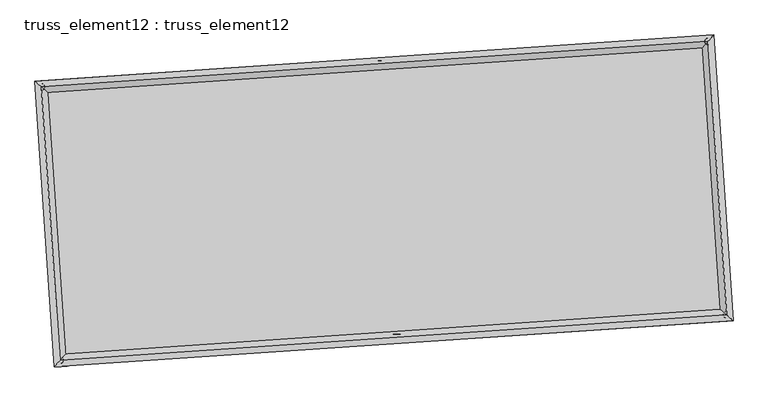
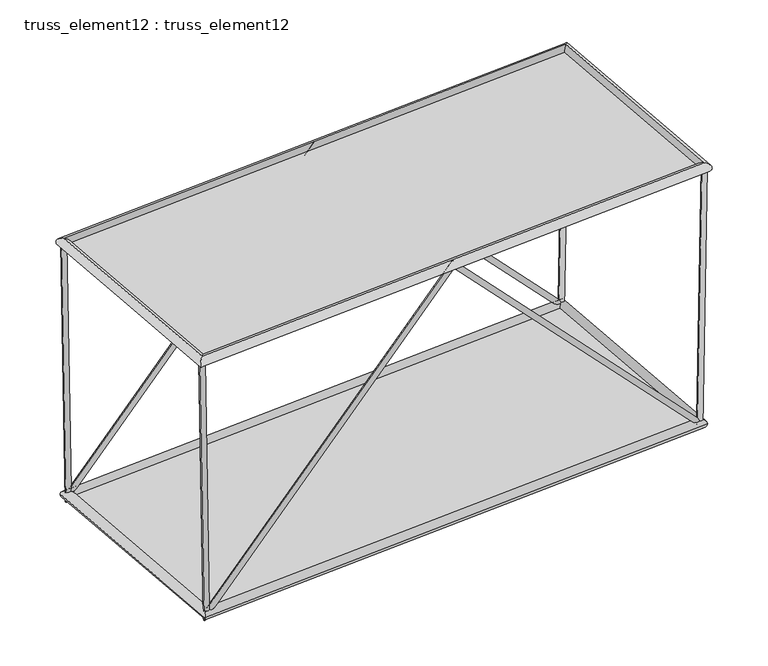
"""IFC4 building model written with IfcOpenShell, lengths in millimetres: plate geometry, truss_element12 : truss_element12."""

import ifcopenshell
import ifcopenshell.guid

model = None  # the IFC model being written
_history = None  # IfcOwnerHistory: only IFC2X3 demands one
_inside = {}  # id of a spatial element -> (the spatial element, [elements in it])
_under = {}  # id of a project, library or spatial element -> (it, [spatial elements below it])
_declared = {}  # id of a project -> (the project, [libraries it declares])
_typed = {}  # id of a type object -> (the type object, [elements of that type])
_made_of = {}  # id of a material, layer set ... -> (it, [elements and type objects made of it])


def new_model(schema):
    """Start an empty IFC model of exactly this schema.

    Asked for "IFC4X3", IfcOpenShell would pick the latest addendum, in which some entities
    have other attributes; the version numbers below select the first issue.
    IFC2X3 requires an IfcOwnerHistory on every rooted entity: one is made here for all.
    """
    global model, _history
    if schema == "IFC4X3":
        model = ifcopenshell.file(schema_version=(4, 3, 0, 0))
    else:
        model = ifcopenshell.file(schema=schema)
    _inside.clear()
    _under.clear()
    _declared.clear()
    _typed.clear()
    _made_of.clear()
    _history = None
    if model.schema == "IFC2X3":
        org = make("IfcOrganization", Name="unknown")
        user = make(
            "IfcPersonAndOrganization",
            ThePerson=make("IfcPerson", FamilyName="unknown"),
            TheOrganization=org,
        )
        app = make(
            "IfcApplication",
            ApplicationDeveloper=org,
            Version="unknown",
            ApplicationFullName="unknown",
            ApplicationIdentifier="unknown",
        )
        _history = make(
            "IfcOwnerHistory",
            OwningUser=user,
            OwningApplication=app,
            ChangeAction="ADDED",
            CreationDate=0,
        )
    return model


def make(cls, **values):
    """One entity of the class cls with the attributes given. An attribute that is None is left unset."""
    return model.create_entity(
        cls, **{name: value for name, value in values.items() if value is not None}
    )


def rooted(cls, **values):
    """An entity with a GlobalId (a new one), such as an element, a storey or a relation."""
    return make(cls, GlobalId=ifcopenshell.guid.new(), OwnerHistory=_history, **values)


def si_unit(unit_type, name, prefix=None):
    """IfcSIUnit, for example si_unit("LENGTHUNIT", "METRE", prefix="MILLI")."""
    return make("IfcSIUnit", UnitType=unit_type, Prefix=prefix, Name=name)


def assignment(units):
    """IfcUnitAssignment: the units of a project."""
    return None if units is None else make("IfcUnitAssignment", Units=units)


def point(xyz):
    """IfcCartesianPoint."""
    return None if xyz is None else make("IfcCartesianPoint", Coordinates=xyz)


def direction(xyz):
    """IfcDirection."""
    return None if xyz is None else make("IfcDirection", DirectionRatios=xyz)


def frame(location, z_axis=None, x_axis=None):
    """IfcAxis2Placement3D, a coordinate frame: its origin and axes. An axis left out is left unset."""
    return make(
        "IfcAxis2Placement3D",
        Location=point(location),
        Axis=direction(z_axis),
        RefDirection=direction(x_axis),
    )


def origin():
    """The frame at (0, 0, 0) with its axes left unset."""
    return frame((0.0, 0.0, 0.0))


def origin_with_axes():
    """The frame at (0, 0, 0) with the z axis (0, 0, 1) and the x axis (1, 0, 0) written out."""
    return frame((0.0, 0.0, 0.0), z_axis=(0.0, 0.0, 1.0), x_axis=(1.0, 0.0, 0.0))


def place(relative_to, where):
    """IfcLocalPlacement: puts the frame where relative to a parent placement (None: the world)."""
    return make(
        "IfcLocalPlacement", PlacementRelTo=relative_to, RelativePlacement=where
    )


def context(
    kind, dimensions, precision=None, world=None, true_north=None, identifier=None
):
    """IfcGeometricRepresentationContext, for example the 3D "Model" context."""
    return make(
        "IfcGeometricRepresentationContext",
        ContextIdentifier=identifier,
        ContextType=kind,
        CoordinateSpaceDimension=dimensions,
        Precision=precision,
        WorldCoordinateSystem=world,
        TrueNorth=true_north,
    )


def project(units=None, contexts=None):
    """IfcProject with its units and contexts."""
    return rooted(
        "IfcProject",
        Name="project",
        RepresentationContexts=contexts,
        UnitsInContext=assignment(units),
    )


def spatial(cls, under=None, at=None, **own):
    """A site, building, storey or space (cls), placed at a placement, below another one or the project."""
    s = rooted(cls, ObjectPlacement=at, **own)
    if under is not None:
        _under.setdefault(under.id(), (under, []))[1].append(s)
    return s


def polyline(points):
    """IfcPolyline through the points."""
    return make("IfcPolyline", Points=[point(p) for p in points])


def circle_curve(where, radius):
    """IfcCircle in the frame where."""
    return make("IfcCircle", Position=where, Radius=radius)


def ellipse_curve(where, semi_axis1, semi_axis2):
    """IfcEllipse in the frame where."""
    return make(
        "IfcEllipse", Position=where, SemiAxis1=semi_axis1, SemiAxis2=semi_axis2
    )


def outline(outer, holes=None, kind="AREA"):
    """IfcArbitraryClosedProfileDef: a profile drawn as a closed curve; with holes, ...WithVoids."""
    if holes is None:
        return make("IfcArbitraryClosedProfileDef", ProfileType=kind, OuterCurve=outer)
    return make(
        "IfcArbitraryProfileDefWithVoids",
        ProfileType=kind,
        OuterCurve=outer,
        InnerCurves=holes,
    )


def extrude(swept, where, along, depth):
    """IfcExtrudedAreaSolid: the profile swept, set in the frame where, extruded along a direction by depth."""
    return make(
        "IfcExtrudedAreaSolid",
        SweptArea=swept,
        Position=where,
        ExtrudedDirection=direction(along),
        Depth=depth,
    )


def shape(context_of_items, identifier, shape_type, items):
    """IfcShapeRepresentation: the items that make up one representation, for example the "Body"."""
    return make(
        "IfcShapeRepresentation",
        ContextOfItems=context_of_items,
        RepresentationIdentifier=identifier,
        RepresentationType=shape_type,
        Items=items,
    )


def source(mapping_origin, context_of_items, identifier, shape_type, items):
    """IfcRepresentationMap: a shape defined once, which mapped items show again and again."""
    return make(
        "IfcRepresentationMap",
        MappingOrigin=mapping_origin,
        MappedRepresentation=shape(context_of_items, identifier, shape_type, items),
    )


def transform(
    local_origin,
    x_axis=None,
    y_axis=None,
    z_axis=None,
    scale=None,
    scale2=None,
    scale3=None,
    uniform=True,
):
    """IfcCartesianTransformationOperator3D, or its non-uniform kind. x_axis, y_axis, z_axis: its Axis1, 2, 3."""
    if uniform:
        return make(
            "IfcCartesianTransformationOperator3D",
            Axis1=direction(x_axis),
            Axis2=direction(y_axis),
            LocalOrigin=point(local_origin),
            Scale=scale,
            Axis3=direction(z_axis),
        )
    return make(
        "IfcCartesianTransformationOperator3DnonUniform",
        Axis1=direction(x_axis),
        Axis2=direction(y_axis),
        LocalOrigin=point(local_origin),
        Scale=scale,
        Axis3=direction(z_axis),
        Scale2=scale2,
        Scale3=scale3,
    )


def mapped(mapping_source, mapping_target):
    """IfcMappedItem: shows the shape of a source again, moved by a transform."""
    return make(
        "IfcMappedItem", MappingSource=mapping_source, MappingTarget=mapping_target
    )


def made_of(thing, what):
    """Note that an element or type object is made of a material, layer set ...; save() writes the relation."""
    if what is not None:
        _made_of.setdefault(what.id(), (what, []))[1].append(thing)
    return thing


def element(
    cls,
    number,
    at=None,
    inside=None,
    cuts=None,
    type_object=None,
    material=None,
    context=None,
    identifier="Body",
    shape_type=None,
    held_by="IfcProductDefinitionShape",
    body=None,
    shapes=None,
    **own,
):
    """One element of the class cls, such as IfcWall. Its Tag is "e" and its number.

    at: its placement. inside: the storey or other place that contains it. cuts: it is an
    opening in that element (IfcRelVoidsElement). A single representation is given by context,
    identifier, shape_type and body (its items); several are given by shapes. held_by: the class
    of the entity that holds the representations. save() writes the other relations.
    """
    e = rooted(cls, Tag="e%d" % number, ObjectPlacement=at, **own)
    if body is not None:
        shapes = [shape(context, identifier, shape_type, body)]
    if shapes is not None:
        e.Representation = make(held_by, Representations=shapes)
    if inside is not None:
        _inside.setdefault(inside.id(), (inside, []))[1].append(e)
    if cuts is not None:
        rooted(
            "IfcRelVoidsElement", RelatingBuildingElement=cuts, RelatedOpeningElement=e
        )
    if type_object is not None:
        _typed.setdefault(type_object.id(), (type_object, []))[1].append(e)
    return made_of(e, material)


def aggregate(whole, parts):
    """IfcRelAggregates: a whole, such as a stair, and the parts it consists of."""
    return rooted("IfcRelAggregates", RelatingObject=whole, RelatedObjects=parts)


def save(model, path):
    """Write the relations noted so far, then the file.

    IfcRelAggregates (storeys below a building ...), IfcRelContainedInSpatialStructure (elements
    in a storey), IfcRelDefinesByType, IfcRelAssociatesMaterial and IfcRelDeclares: one each for
    every whole, place, type object, material and project.
    """
    for whole, parts in _under.values():
        aggregate(whole, parts)
    for where, things in _inside.values():
        rooted(
            "IfcRelContainedInSpatialStructure",
            RelatedElements=things,
            RelatingStructure=where,
        )
    for kind, things in _typed.values():
        rooted("IfcRelDefinesByType", RelatedObjects=things, RelatingType=kind)
    for what, things in _made_of.values():
        rooted("IfcRelAssociatesMaterial", RelatedObjects=things, RelatingMaterial=what)
    for by, libraries in _declared.values():
        rooted("IfcRelDeclares", RelatingContext=by, RelatedDefinitions=libraries)
    model.write(path)


def plane_surface(at):
    """IfcPlane: the flat surface through the origin of the frame at, square to its z axis."""
    return make("IfcPlane", Position=at)


def cylinder_surface(at, radius):
    """IfcCylindricalSurface: all points at the distance radius from the z axis of the frame at."""
    return make("IfcCylindricalSurface", Position=at, Radius=radius)


def advanced_brep(points, edges, surfaces, faces):
    """IfcAdvancedBrep: a solid bounded by faces that lie on surfaces and meet in shared edges.

    An edge is (start, end): straight between two places in points (the first is 0);
    or (start, end, curve); or (start, end, curve, False) where it runs against its curve.
    A face is (place in surfaces, loops), or (place, loops, False) where it looks against
    its surface's normal. A loop lists edges by number (the first is 1), with a minus sign
    where the edge is run from its end to its start. The first loop is the outer one.
    """
    corners = [point(p) for p in points]
    vertices = [make("IfcVertexPoint", VertexGeometry=c) for c in corners]
    made = []
    for start, end, *more in edges:
        made.append(
            make(
                "IfcEdgeCurve",
                EdgeStart=vertices[start],
                EdgeEnd=vertices[end],
                EdgeGeometry=more[0] if more else make("IfcPolyline", Points=[corners[start], corners[end]]),
                SameSense=more[1] if len(more) > 1 else True,
            )
        )
    hull = []
    for where, loops, *sense in faces:
        bounds = []
        for j, loop in enumerate(loops):
            ring = [make("IfcOrientedEdge", EdgeElement=made[abs(k) - 1], Orientation=k > 0) for k in loop]
            bounds.append(
                make(
                    "IfcFaceOuterBound" if j == 0 else "IfcFaceBound",
                    Bound=make("IfcEdgeLoop", EdgeList=ring),
                    Orientation=True,
                )
            )
        hull.append(make("IfcAdvancedFace", Bounds=bounds, FaceSurface=surfaces[where], SameSense=sense[0] if sense else True))
    return make("IfcAdvancedBrep", Outer=make("IfcClosedShell", CfsFaces=hull))


def truss_element12_truss_element12_d2dc27e5(model_context):
    return source(origin(), model_context, "Body", "SolidModel", [
        advanced_brep(
        [(-3750.4936923, 2270.3904911, 5000.120325), (-3849.582422, 2257.0302647, 4998.409186), (-3667.0221146, 2276.0821006, 122.0048198), (-3761.9647682, 2263.0045795, -122.0048198), (1064.434046, 2598.7021103, 5071.3707956), (1064.871576, 2592.1282012, 4927.1341263), (5794.4951758, 2921.2269981, 121.9949961), (5890.2658012, 2921.1534904, -121.9949961), (5879.3513588, 2927.0130186, 5000.1099238), (5979.3359995, 2927.2268486, 4998.3704092)],
        [
            (0, 1, circle_curve(frame((-3800.0380572, 2263.7103779, 4999.2647555), z_axis=(-0.01710892315204124, -0.0011665924326349144, 0.9998529510936465), x_axis=(-0.13360257959464636, 0.9910343456266016, -0.00112982923926399)), 50.0)),
            (1, 0, circle_curve(frame((-3800.0380572, 2263.7103779, 4999.2647555), z_axis=(-0.01710892315204124, -0.0011665924326349144, 0.9998529510936465), x_axis=(-0.13360257959464636, 0.9910343456266016, -0.00112982923926399)), 50.0)),
            (0, 2),
            (2, 3, ellipse_curve(frame((-3714.4934414, 2269.54334, 0.0), z_axis=(-0.9289170101606278, -0.06333931977871671, 0.3648305343638462), x_axis=(0.36398536651593416, 0.024818778504806103, 0.9310739397039263)), 131.3219892, 50.0)),
            (3, 1),
            (3, 2, ellipse_curve(frame((-3714.4934414, 2269.54334, 0.0), z_axis=(-0.9289170101606278, -0.06333931977871671, 0.3648305343638462), x_axis=(0.36398536651593416, 0.024818778504806103, 0.9310739397039263)), 131.3219892, 50.0)),
            (2, 4),
            (4, 5, ellipse_curve(frame((1064.652811, 2595.4151558, 4999.252461), z_axis=(-0.9976833933321771, -0.06802823804168875, 7.414941499714515e-05), x_axis=(-7.39776401714257e-05, -5.0442540650833885e-06, -0.9999999972509322)), 72.2753704, 50.0)),
            (5, 3),
            (5, 4, ellipse_curve(frame((1064.652811, 2595.4151558, 4999.252461), z_axis=(-0.9976833933321771, -0.06802823804168875, 7.414941499714515e-05), x_axis=(-7.39776401714257e-05, -5.0442540650833885e-06, -0.9999999972509322)), 72.2753704, 50.0)),
            (4, 6),
            (6, 7, ellipse_curve(frame((5842.3804885, 2921.1902443, 0.0), z_axis=(-0.9289957394028395, -0.06334468802646322, -0.3646290809441854), x_axis=(-0.36378437978405576, -0.02480507398358674, 0.931152851754103)), 131.300287, 50.0)),
            (7, 5),
            (7, 6, ellipse_curve(frame((5842.3804885, 2921.1902443, 0.0), z_axis=(-0.9289957394028395, -0.06334468802646322, -0.3646290809441854), x_axis=(-0.36378437978405576, -0.02480507398358674, 0.931152851754103)), 131.300287, 50.0)),
            (8, 9, circle_curve(frame((5929.3436792, 2927.1199336, 4999.2401665), z_axis=(0.017392638132466113, 0.001185937878642774, 0.9998480332981313), x_axis=(-0.002158604726762429, 0.9999970106075159, -0.0011485650461673309)), 50.0)),
            (9, 8, circle_curve(frame((5929.3436792, 2927.1199336, 4999.2401665), z_axis=(0.017392638132466113, 0.001185937878642774, 0.9998480332981313), x_axis=(-0.002158604726762429, 0.9999970106075159, -0.0011485650461673309)), 50.0)),
            (6, 8),
            (9, 7),
        ],
        [
            plane_surface(frame((-3800.0380572, 2313.7103439, 4999.3230936), z_axis=(-0.01710892315204017, -0.001166592432634736, 0.9998529510936465), x_axis=(0.9998536316624437, -1.9962062093981113e-05, 0.017108911506536383))),
            cylinder_surface(frame((-3800.0380572, 2263.7103779, 4999.2647555), z_axis=(-0.017108923152041242, -0.0011665924326349146, 0.9998529510936467), x_axis=(-0.13360257959464636, 0.9910343456266016, -0.00112982923926399)), 50.0),
            cylinder_surface(frame((-3714.4934414, 2269.54334, 0.0), z_axis=(-0.69024939212398, -0.04706548216534755, -0.7220392074264527), x_axis=(-0.020419483033555893, 0.998751870731873, -0.045582292858373695)), 50.0),
            cylinder_surface(frame((1064.652811, 2595.4151558, 4999.252461), z_axis=(-0.6901425550207504, -0.04705819734940832, 0.7221418003492492), x_axis=(-0.11534812165123533, 0.9922790477220719, -0.045575237611120895)), 50.0),
            plane_surface(frame((5929.3436792, 2877.1199688, 4999.2994724), z_axis=(0.01739263813246562, 0.001185937878642426, 0.9998480332981314), x_axis=(0.9998487366290929, -2.0629708890496073e-05, -0.017392625897834066))),
            cylinder_surface(frame((5842.3804885, 2921.1902443, 0.0), z_axis=(-0.017392638132466113, -0.001185937878642774, -0.9998480332981313), x_axis=(-0.002158604726762429, 0.9999970106075159, -0.0011485650461673309)), 50.0),
        ],
        [
            (0, [[1, 2]]),
            (1, [[-1, 3, 4, 5]]),
            (1, [[-2, -5, 6, -3]]),
            (2, [[-4, 7, 8, 9]]),
            (2, [[-6, -9, 10, -7]]),
            (3, [[-8, 11, 12, 13]]),
            (3, [[-10, -13, 14, -11]]),
            (4, [[15, 16]]),
            (5, [[-12, 17, -16, 18]]),
            (5, [[-14, -18, -15, -17]]),
        ],
    ),
        advanced_brep(
        [(-3478.3807394, -1720.3430932, 5000.120325), (-3577.4694691, -1733.7033196, 4998.409186), (-3394.9091617, -1714.6514837, 122.0048198), (-3489.8518153, -1727.7290048, -122.0048198), (1336.5469989, -1392.031474, 5071.3707956), (1336.9845289, -1398.6053831, 4927.1341263), (6066.6081287, -1069.5065862, 121.9949961), (6162.3787541, -1069.5800939, -121.9949961), (6151.4643118, -1063.7205657, 5000.1099238), (6251.4489524, -1063.5067356, 4998.3704092)],
        [
            (0, 1, circle_curve(frame((-3527.9251043, -1727.0232064, 4999.2647555), z_axis=(-0.017108923152041454, -0.0011665924326349345, 0.9998529510936464), x_axis=(-0.1336025795946458, 0.9910343456266016, -0.0011298292392639894)), 50.0)),
            (1, 0, circle_curve(frame((-3527.9251043, -1727.0232064, 4999.2647555), z_axis=(-0.017108923152041454, -0.0011665924326349345, 0.9998529510936464), x_axis=(-0.1336025795946458, 0.9910343456266016, -0.0011298292392639894)), 50.0)),
            (0, 2),
            (2, 3, ellipse_curve(frame((-3442.3804885, -1721.1902443, 0.0), z_axis=(-0.9289170101606279, -0.06333931977871649, 0.36483053436384594), x_axis=(0.36398536651593394, 0.024818778504805978, 0.9310739397039264)), 131.3219892, 50.0)),
            (3, 1),
            (3, 2, ellipse_curve(frame((-3442.3804885, -1721.1902443, 0.0), z_axis=(-0.9289170101606279, -0.06333931977871649, 0.36483053436384594), x_axis=(0.36398536651593394, 0.024818778504805978, 0.9310739397039264)), 131.3219892, 50.0)),
            (2, 4),
            (4, 5, ellipse_curve(frame((1336.7657639, -1395.3184285, 4999.252461), z_axis=(-0.9976833933321771, -0.0680282380416885, 7.414941499714518e-05), x_axis=(-7.397764017142569e-05, -5.0442540650641685e-06, -0.9999999972509322)), 72.2753704, 50.0)),
            (5, 3),
            (5, 4, ellipse_curve(frame((1336.7657639, -1395.3184285, 4999.252461), z_axis=(-0.9976833933321771, -0.0680282380416885, 7.414941499714518e-05), x_axis=(-7.397764017142569e-05, -5.0442540650641685e-06, -0.9999999972509322)), 72.2753704, 50.0)),
            (4, 6),
            (6, 7, ellipse_curve(frame((6114.4934414, -1069.54334, 0.0), z_axis=(-0.9289957394028399, -0.06334468802646308, -0.3646290809441853), x_axis=(-0.36378437978405553, -0.02480507398358664, 0.9311528517541031)), 131.300287, 50.0)),
            (7, 5),
            (7, 6, ellipse_curve(frame((6114.4934414, -1069.54334, 0.0), z_axis=(-0.9289957394028399, -0.06334468802646308, -0.3646290809441853), x_axis=(-0.36378437978405553, -0.02480507398358664, 0.9311528517541031)), 131.300287, 50.0)),
            (8, 9, circle_curve(frame((6201.4566321, -1063.6136507, 4999.2401665), z_axis=(0.01739263813246659, 0.0011859378786428217, 0.9998480332981314), x_axis=(-0.00215860472676268, 0.999997010607516, -0.0011485650461673731)), 50.0)),
            (9, 8, circle_curve(frame((6201.4566321, -1063.6136507, 4999.2401665), z_axis=(0.01739263813246659, 0.0011859378786428217, 0.9998480332981314), x_axis=(-0.00215860472676268, 0.999997010607516, -0.0011485650461673731)), 50.0)),
            (6, 8),
            (9, 7),
        ],
        [
            plane_surface(frame((-3527.9251043, -1677.0232404, 4999.3230936), z_axis=(-0.01710892315204017, -0.0011665924326347264, 0.9998529510936465), x_axis=(0.9998536316624437, -1.9962062093981113e-05, 0.017108911506536383))),
            cylinder_surface(frame((-3527.9251043, -1727.0232064, 4999.2647555), z_axis=(-0.017108923152041457, -0.0011665924326349348, 0.9998529510936466), x_axis=(-0.1336025795946458, 0.9910343456266016, -0.0011298292392639894)), 50.0),
            cylinder_surface(frame((-3442.3804885, -1721.1902443, 0.0), z_axis=(-0.6902493921239796, -0.04706548216534734, -0.7220392074264529), x_axis=(-0.02041948303355586, 0.998751870731873, -0.04558229285837343)), 50.0),
            cylinder_surface(frame((1336.7657639, -1395.3184285, 4999.252461), z_axis=(-0.6901425550207501, -0.04705819734940815, 0.7221418003492494), x_axis=(-0.11534812165123483, 0.9922790477220719, -0.04557523761112062)), 50.0),
            plane_surface(frame((6201.4566321, -1113.6136155, 4999.2994724), z_axis=(0.01739263813246562, 0.0011859378786424177, 0.9998480332981314), x_axis=(0.9998487366290929, -2.0629708890051984e-05, -0.017392625897834066))),
            cylinder_surface(frame((6114.4934414, -1069.54334, 0.0), z_axis=(-0.01739263813246659, -0.0011859378786428217, -0.9998480332981314), x_axis=(-0.00215860472676268, 0.999997010607516, -0.0011485650461673731)), 50.0),
        ],
        [
            (0, [[1, 2]]),
            (1, [[-1, 3, 4, 5]]),
            (1, [[-2, -5, 6, -3]]),
            (2, [[-4, 7, 8, 9]]),
            (2, [[-6, -9, 10, -7]]),
            (3, [[-8, 11, 12, 13]]),
            (3, [[-10, -13, 14, -11]]),
            (4, [[15, 16]]),
            (5, [[-12, 17, -16, 18]]),
            (5, [[-14, -18, -15, -17]]),
        ],
    ),
        advanced_brep(
        [(-3527.9315258, -1727.0303236, 4909.2647557), (-3527.9186827, -1727.0160892, 5089.2647552), (-3800.030729, 2263.7041982, 5089.2647552), (-3800.0453854, 2263.7165576, 4909.2647557), (5929.3377104, 2927.1128473, 5089.2401663), (5929.3496479, 2927.12702, 4909.2401667), (6201.4497567, -1063.6074401, 5089.2401663), (6201.4635075, -1063.6198612, 4909.2401667)],
        [
            (0, 1, ellipse_curve(frame((-3527.9251043, -1727.0232064, 4999.2647555), z_axis=(-0.7535719234032141, 0.6573654662782353, 1.7829245935204696e-06), x_axis=(-0.6573654662758399, -0.7535719234053034, 1.7829245812694147e-06)), 127.2792206, 90.0)),
            (1, 2),
            (2, 3, ellipse_curve(frame((-3800.0380572, 2263.7103779, 4999.2647555), z_axis=(-0.6573654662758396, -0.753571923405304, 1.7829245811910703e-06), x_axis=(0.7535719234032143, -0.6573654662782349, -1.7829245934421267e-06)), 127.2792206, 90.0)),
            (3, 0),
            (1, 0, ellipse_curve(frame((-3527.9251043, -1727.0232064, 4999.2647555), z_axis=(-0.7535719234032141, 0.6573654662782353, 1.7829245935204696e-06), x_axis=(-0.6573654662758399, -0.7535719234053034, 1.7829245812694147e-06)), 127.2792206, 90.0)),
            (3, 2, ellipse_curve(frame((-3800.0380572, 2263.7103779, 4999.2647555), z_axis=(-0.6573654662758396, -0.753571923405304, 1.7829245811910703e-06), x_axis=(0.7535719234032143, -0.6573654662782349, -1.7829245934421267e-06)), 127.2792206, 90.0)),
            (2, 4),
            (4, 5, ellipse_curve(frame((5929.3436792, 2927.1199336, 4999.2401665), z_axis=(-0.7535719234032134, 0.6573654662782358, 1.782924593633729e-06), x_axis=(-0.6573654662758406, -0.753571923405303, 1.7829245809994683e-06)), 127.2792206, 90.0)),
            (5, 3),
            (5, 4, ellipse_curve(frame((5929.3436792, 2927.1199336, 4999.2401665), z_axis=(-0.7535719234032134, 0.6573654662782358, 1.782924593633729e-06), x_axis=(-0.6573654662758406, -0.753571923405303, 1.7829245809994683e-06)), 127.2792206, 90.0)),
            (4, 6),
            (6, 7, ellipse_curve(frame((6201.4566321, -1063.6136507, 4999.2401665), z_axis=(0.6573654662758406, 0.7535719234053031, -1.7829245810778119e-06), x_axis=(-0.7535719234032136, 0.6573654662782359, 1.7829245937120725e-06)), 127.2792206, 90.0)),
            (7, 5),
            (7, 6, ellipse_curve(frame((6201.4566321, -1063.6136507, 4999.2401665), z_axis=(0.6573654662758406, 0.7535719234053031, -1.7829245810778119e-06), x_axis=(-0.7535719234032136, 0.6573654662782359, 1.7829245937120725e-06)), 127.2792206, 90.0)),
            (6, 1),
            (0, 7),
        ],
        [
            cylinder_surface(frame((-3527.9251043, -1727.0232064, 4999.2647555), z_axis=(0.06802823822869955, -0.9976833960748767, 0.0), x_axis=(-0.9976833931505921, -0.0680282380293037, 7.65646749386812e-05)), 90.0),
            cylinder_surface(frame((-3800.0380572, 2263.7103779, 4999.2647555), z_axis=(-0.9976833960717053, -0.06802823822848321, 2.5214361320715873e-06), x_axis=(-0.06802823785595762, 0.9976833933527269, 7.404323882218444e-05)), 90.0),
            cylinder_surface(frame((5929.3436792, 2927.1199336, 4999.2401665), z_axis=(-0.06802823822869739, 0.997683396074877, 0.0), x_axis=(0.997683393523118, 0.06802823805470264, 7.152180268809107e-05)), 90.0),
            cylinder_surface(frame((6201.4566321, -1063.6136507, 4999.2401665), z_axis=(0.9976833960717054, 0.06802823822848272, -2.5214361321823818e-06), x_axis=(0.06802823822848272, -0.9976833933273259, 7.404323880442816e-05)), 90.0),
        ],
        [
            (0, [[1, 2, 3, 4]]),
            (0, [[5, -4, 6, -2]]),
            (1, [[-3, 7, 8, 9]]),
            (1, [[-6, -9, 10, -7]]),
            (2, [[-8, 11, 12, 13]]),
            (2, [[-10, -13, 14, -11]]),
            (3, [[-12, 15, -1, 16]]),
            (3, [[-14, -16, -5, -15]]),
        ],
    ),
        advanced_brep(
        [(-3358.7115243, -1625.2761972, 0.0), (-3526.0494527, -1817.1042913, 0.0), (-3810.4074885, 2353.2123043, 0.0), (-3618.5793943, 2185.8743758, 0.0), (5926.0494527, 3017.1042913, 0.0), (5758.7115243, 2825.2761972, 0.0), (6210.4074885, -1153.2123043, 0.0), (6018.5793943, -985.8743758, 0.0)],
        [
            (0, 1, ellipse_curve(frame((-3442.3804885, -1721.1902443, 0.0), z_axis=(-0.7535719234054589, 0.6573654662780798, 0.0), x_axis=(-0.6573654662780798, -0.7535719234054589, 0.0)), 127.2792206, 90.0)),
            (1, 2),
            (2, 3, ellipse_curve(frame((-3714.4934414, 2269.54334, 0.0), z_axis=(-0.6573654662780795, -0.753571923405459, 0.0), x_axis=(0.7535719234054589, -0.6573654662780798, 0.0)), 127.2792206, 90.0)),
            (3, 0),
            (1, 0, ellipse_curve(frame((-3442.3804885, -1721.1902443, 0.0), z_axis=(-0.7535719234054589, 0.6573654662780798, 0.0), x_axis=(-0.6573654662780798, -0.7535719234054589, 0.0)), 127.2792206, 90.0)),
            (3, 2, ellipse_curve(frame((-3714.4934414, 2269.54334, 0.0), z_axis=(-0.6573654662780795, -0.753571923405459, 0.0), x_axis=(0.7535719234054589, -0.6573654662780798, 0.0)), 127.2792206, 90.0)),
            (2, 4),
            (4, 5, ellipse_curve(frame((5842.3804885, 2921.1902443, 0.0), z_axis=(-0.7535719234054582, 0.6573654662780805, 0.0), x_axis=(-0.6573654662780805, -0.7535719234054581, 0.0)), 127.2792206, 90.0)),
            (5, 3),
            (5, 4, ellipse_curve(frame((5842.3804885, 2921.1902443, 0.0), z_axis=(-0.7535719234054582, 0.6573654662780805, 0.0), x_axis=(-0.6573654662780805, -0.7535719234054581, 0.0)), 127.2792206, 90.0)),
            (4, 6),
            (6, 7, ellipse_curve(frame((6114.4934414, -1069.54334, 0.0), z_axis=(0.6573654662780807, 0.7535719234054581, 0.0), x_axis=(-0.7535719234054581, 0.6573654662780806, 0.0)), 127.2792206, 90.0)),
            (7, 5),
            (7, 6, ellipse_curve(frame((6114.4934414, -1069.54334, 0.0), z_axis=(0.6573654662780807, 0.7535719234054581, 0.0), x_axis=(-0.7535719234054581, 0.6573654662780806, 0.0)), 127.2792206, 90.0)),
            (6, 1),
            (0, 7),
        ],
        [
            cylinder_surface(frame((-3442.3804885, -1721.1902443, 0.0), z_axis=(0.06802823822870281, -0.9976833960748764, 0.0), x_axis=(-0.9976833960748764, -0.06802823822870281, 0.0)), 90.0),
            cylinder_surface(frame((-3714.4934414, 2269.54334, 0.0), z_axis=(-0.9976833960748764, -0.06802823822870283, 0.0), x_axis=(-0.06802823822870283, 0.9976833960748764, 0.0)), 90.0),
            cylinder_surface(frame((5842.3804885, 2921.1902443, 0.0), z_axis=(-0.06802823822870042, 0.9976833960748767, 0.0), x_axis=(0.9976833960748767, 0.06802823822870042, 0.0)), 90.0),
            cylinder_surface(frame((6114.4934414, -1069.54334, 0.0), z_axis=(0.9976833960748765, 0.06802823822870231, 0.0), x_axis=(0.06802823822870231, -0.9976833960748765, 0.0)), 90.0),
        ],
        [
            (0, [[1, 2, 3, 4]]),
            (0, [[5, -4, 6, -2]]),
            (1, [[-3, 7, 8, 9]]),
            (1, [[-6, -9, 10, -7]]),
            (2, [[-8, 11, 12, 13]]),
            (2, [[-10, -13, 14, -11]]),
            (3, [[-12, 15, -1, 16]]),
            (3, [[-14, -16, -5, -15]]),
        ],
    ),
        extrude(outline(polyline([(-3442.3804885, -1721.1902443), (-3714.4934414, 2269.54334), (5842.3804885, 2921.1902443), (6114.4934414, -1069.54334), (-3442.3804885, -1721.1902443)])), origin_with_axes(), (0.0, 0.0, 1.0), 20.0),
        extrude(outline(polyline([(-2000.0, 4875.986598), (2000.0, 4875.9865979), (2000.0, -4875.9865979), (-2000.0, -4875.9865978), (-2000.0, 4875.986598)])), frame((1200.7092875, 600.0483636, 4999.252461), z_axis=(2.515594963820283e-06, 1.7152884922814844e-07, 0.9999999999968212), x_axis=(-0.06802823822870298, 0.9976833960748764, 0.0)), (0.0, 0.0, 1.0), 20.0),
    ])


if __name__ == "__main__":
    model = new_model("IFC4")
    model_context = context("Model", 3, world=origin())
    ifc_project = project(units=[si_unit("LENGTHUNIT", "METRE", prefix="MILLI")], contexts=[model_context])
    site = spatial("IfcSite", under=ifc_project)
    building = spatial("IfcBuilding", under=site)
    placement = place(None, origin())
    truss_element12_truss_element12_shape = truss_element12_truss_element12_d2dc27e5(model_context)
    element("IfcPlate", 1, ObjectType="truss_element12 : truss_element12", at=placement, inside=building, context=model_context, shape_type="MappedRepresentation", body=[
        mapped(truss_element12_truss_element12_shape, transform((0.0, 0.0, 0.0), x_axis=(1.0, 0.0, 0.0), y_axis=(0.0, 1.0, 0.0), z_axis=(0.0, 0.0, 1.0))),
    ])
    save(model, "model.ifc")

# Revit data of these elements
# Type "truss_element12 : truss_element12"
#   steellbar1 = 90 mm
#   steelbar2 = 50 mm
#   offset1 = 5000 mm
#   M = Default Roof
# Element 1 (IfcPlate, "truss_element12 : truss_element12")
#   Materials on its faces: "Default Roof"
# Materials
#   "Default Roof": class "Miscellaneous", colour RGB 0 127 0, transparency 0, Comments = "Rendering appearance not upgraded Rendering appearance not upgraded ", Cost = 0
